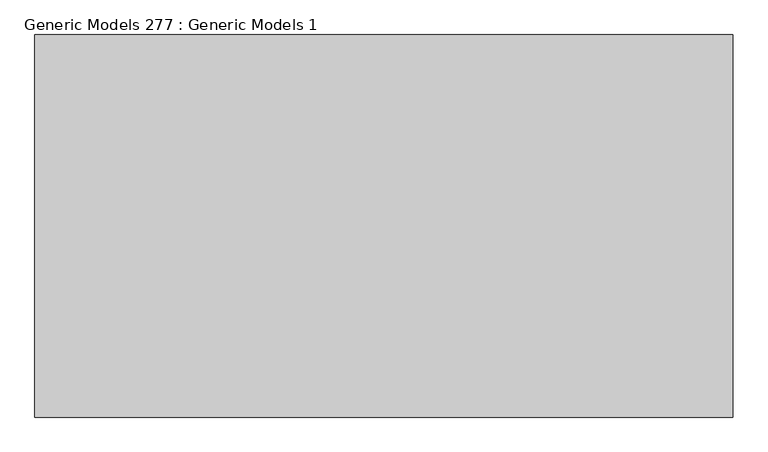
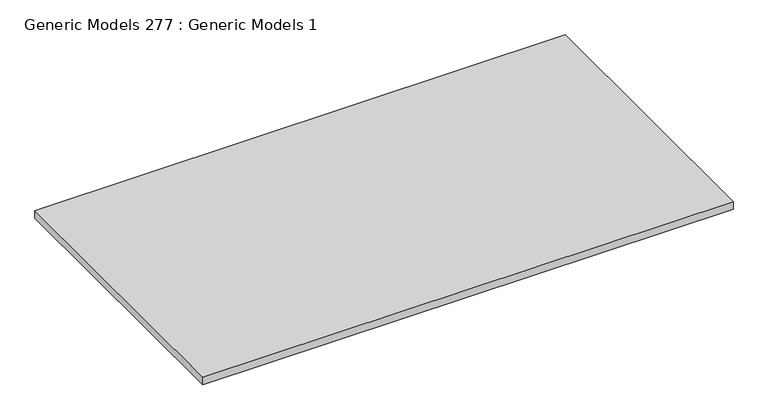
"""IFC4 building model written with IfcOpenShell, lengths in millimetres: proxy geometry, Generic Models 277 : Generic Models 1."""

from ifc_helpers import new_model, si_unit, frame, origin, place, context, project, spatial, polyline, outline, extrude, source, transform, mapped, element, save


def generic_models_277_generic_models_1_51c903ee(model_context):
    return source(origin(), model_context, "Body", "SweptSolid", [
        extrude(outline(polyline([(3342.6963858, 1085.2769662), (4593.7023574, 1085.2769662), (4593.7023574, 399.7309662), (3342.6963858, 399.7309662), (3342.6963858, 1085.2769662)])), frame((0.0, 0.0, 126783.846), z_axis=(0.0, 0.0, 1.0), x_axis=(1.0, 0.0, 0.0)), (0.0, 0.0, 1.0), 19.05),
    ])


if __name__ == "__main__":
    model = new_model("IFC4")
    model_context = context("Model", 3, world=origin())
    ifc_project = project(units=[si_unit("LENGTHUNIT", "METRE", prefix="MILLI")], contexts=[model_context])
    site = spatial("IfcSite", under=ifc_project)
    building = spatial("IfcBuilding", under=site)
    placement = place(None, origin())
    generic_models_277_generic_models_1_shape = generic_models_277_generic_models_1_51c903ee(model_context)
    element("IfcBuildingElementProxy", 1, Name="Generic Models 277 : Generic Models 1", ObjectType="Generic Models 277 : Generic Models 1", at=placement, inside=building, context=model_context, shape_type="MappedRepresentation", body=[
        mapped(generic_models_277_generic_models_1_shape, transform((0.0, 0.0, 0.0), x_axis=(1.0, 0.0, 0.0), y_axis=(0.0, 1.0, 0.0), z_axis=(0.0, 0.0, 1.0))),
    ])
    save(model, "model.ifc")

# Revit data of these elements
# Element 1 (IfcBuildingElementProxy, "Generic Models 277 : Generic Models 1")
#   Materials on its faces: "_CDX PLYWOOD - SEE STRUCT DWGs"
# Materials
#   "_CDX PLYWOOD - SEE STRUCT DWGs": class "Generic", colour RGB 98 75 74, transparency 0, Cost = 0
